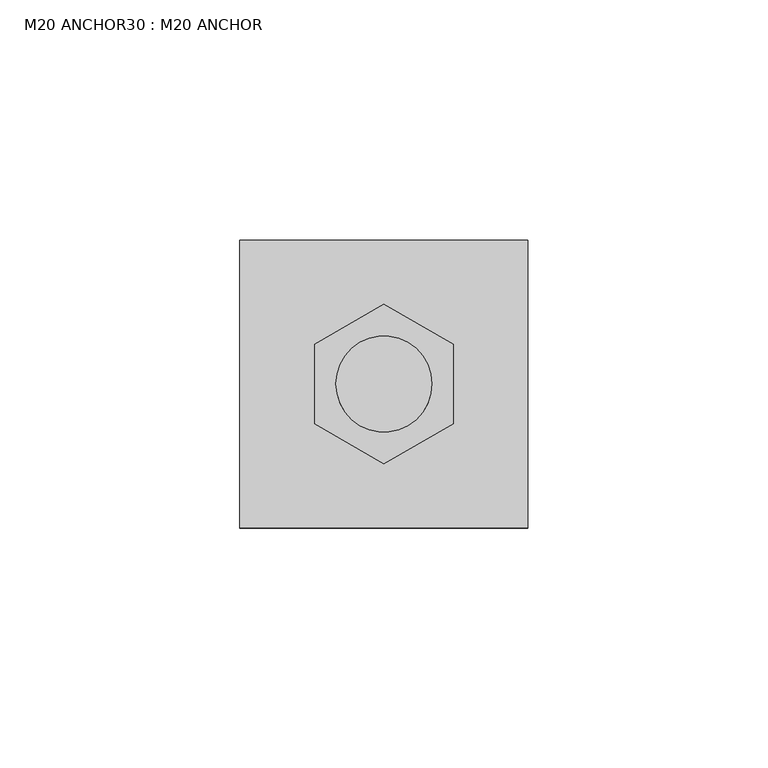
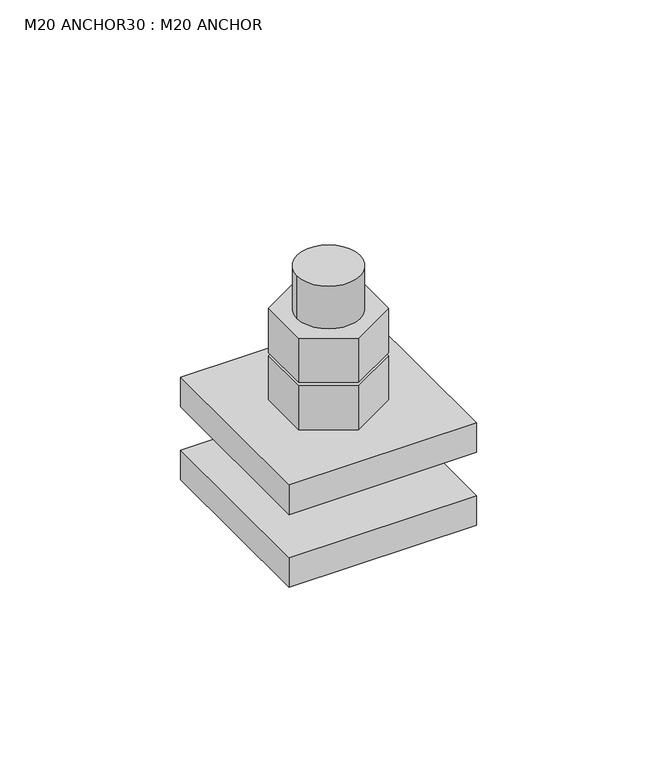
"""IFC4 building model written with IfcOpenShell, lengths in millimetres: fastener geometry, M20 ANCHOR30 : M20 ANCHOR."""

from ifc_helpers import new_model, si_unit, point, frame, frame_2d, origin, place, context, project, spatial, polyline, circle_curve, trimmed, segment, composite_curve, outline, extrude, source, transform, mapped, element, save


def m20_anchor30_m20_anchor_81d38608(model_context):
    return source(origin(), model_context, "Body", "SweptSolid", [
        extrude(outline(polyline([(-30872.0439916, -7426.8093347), (-30886.4521106, -7435.1278661), (-30900.8602297, -7426.8093347), (-30900.8602297, -7410.1722719), (-30886.4521106, -7401.8537405), (-30872.0439916, -7410.1722719), (-30872.0439916, -7426.8093347)]), holes=[composite_curve([segment(trimmed(circle_curve(frame_2d((-30886.4521106, -7418.4908033)), 10.0), [point((-30896.4521106, -7418.4908033))], [point((-30876.4521106, -7418.4908033))], True, "CARTESIAN"), True, "CONTINUOUS"), segment(trimmed(circle_curve(frame_2d((-30886.4521106, -7418.4908033)), 10.0), [point((-30876.4521106, -7418.4908033))], [point((-30896.4521106, -7418.4908033))], True, "CARTESIAN"), True, "CONTINUOUS")], self_intersect=False)]), frame((0.0, 0.0, 240.6), z_axis=(0.0, 0.0, 1.0), x_axis=(1.0, 0.0, 0.0)), (0.0, 0.0, 1.0), 15.0),
        extrude(outline(polyline([(-30872.0439916, -7426.8093347), (-30886.4521106, -7435.1278661), (-30900.8602297, -7426.8093347), (-30900.8602297, -7410.1722719), (-30886.4521106, -7401.8537405), (-30872.0439916, -7410.1722719), (-30872.0439916, -7426.8093347)]), holes=[composite_curve([segment(trimmed(circle_curve(frame_2d((-30886.4521106, -7418.4908033)), 10.0), [point((-30896.4521106, -7418.4908033))], [point((-30876.4521106, -7418.4908033))], True, "CARTESIAN"), True, "CONTINUOUS"), segment(trimmed(circle_curve(frame_2d((-30886.4521106, -7418.4908033)), 10.0), [point((-30876.4521106, -7418.4908033))], [point((-30896.4521106, -7418.4908033))], True, "CARTESIAN"), True, "CONTINUOUS")], self_intersect=False)]), frame((0.0, 0.0, 224.6), z_axis=(0.0, 0.0, 1.0), x_axis=(1.0, 0.0, 0.0)), (0.0, 0.0, 1.0), 15.0),
        extrude(outline(composite_curve([segment(trimmed(circle_curve(frame_2d((-30886.4521106, -7418.4908033)), 10.0), [point((-30896.4521106, -7418.4908033))], [point((-30876.4521106, -7418.4908033))], False, "CARTESIAN"), True, "CONTINUOUS"), segment(trimmed(circle_curve(frame_2d((-30886.4521106, -7418.4908033)), 10.0), [point((-30876.4521106, -7418.4908033))], [point((-30896.4521106, -7418.4908033))], False, "CARTESIAN"), True, "CONTINUOUS")], self_intersect=False)), frame((0.0, 0.0, 190.0), z_axis=(0.0, 0.0, 1.0), x_axis=(1.0, 0.0, 0.0)), (0.0, 0.0, 1.0), 80.0),
        extrude(outline(polyline([(-30856.4521106, -7448.4908033), (-30916.4521106, -7448.4908033), (-30916.4521106, -7388.4908033), (-30856.4521106, -7388.4908033), (-30856.4521106, -7448.4908033)]), holes=[composite_curve([segment(trimmed(circle_curve(frame_2d((-30886.4521106, -7418.4908033)), 11.0), [point((-30897.4521106, -7418.4908033))], [point((-30875.4521106, -7418.4908033))], True, "CARTESIAN"), True, "CONTINUOUS"), segment(trimmed(circle_curve(frame_2d((-30886.4521106, -7418.4908033)), 11.0), [point((-30875.4521106, -7418.4908033))], [point((-30897.4521106, -7418.4908033))], True, "CARTESIAN"), True, "CONTINUOUS")], self_intersect=False)]), frame((0.0, 0.0, 190.0), z_axis=(0.0, 0.0, 1.0), x_axis=(1.0, 0.0, 0.0)), (0.0, 0.0, 1.0), 10.0),
        extrude(outline(polyline([(-30856.4521106, -7448.4908033), (-30916.4521106, -7448.4908033), (-30916.4521106, -7388.4908033), (-30856.4521106, -7388.4908033), (-30856.4521106, -7448.4908033)]), holes=[composite_curve([segment(trimmed(circle_curve(frame_2d((-30886.4521106, -7418.4908033)), 11.0), [point((-30897.4521106, -7418.4908033))], [point((-30875.4521106, -7418.4908033))], True, "CARTESIAN"), True, "CONTINUOUS"), segment(trimmed(circle_curve(frame_2d((-30886.4521106, -7418.4908033)), 11.0), [point((-30875.4521106, -7418.4908033))], [point((-30897.4521106, -7418.4908033))], True, "CARTESIAN"), True, "CONTINUOUS")], self_intersect=False)]), frame((0.0, 0.0, 214.6), z_axis=(0.0, 0.0, 1.0), x_axis=(1.0, 0.0, 0.0)), (0.0, 0.0, 1.0), 10.0),
    ])


if __name__ == "__main__":
    model = new_model("IFC4")
    model_context = context("Model", 3, world=origin())
    ifc_project = project(units=[si_unit("LENGTHUNIT", "METRE", prefix="MILLI")], contexts=[model_context])
    site = spatial("IfcSite", under=ifc_project)
    building = spatial("IfcBuilding", under=site)
    placement = place(None, origin())
    m20_anchor30_m20_anchor_shape = m20_anchor30_m20_anchor_81d38608(model_context)
    element("IfcFastener", 1, ObjectType="M20 ANCHOR30 : M20 ANCHOR", at=placement, inside=building, context=model_context, shape_type="MappedRepresentation", body=[
        mapped(m20_anchor30_m20_anchor_shape, transform((0.0, 0.0, 0.0), x_axis=(1.0, 0.0, 0.0), y_axis=(0.0, 1.0, 0.0), z_axis=(0.0, 0.0, 1.0))),
    ])
    save(model, "model.ifc")
